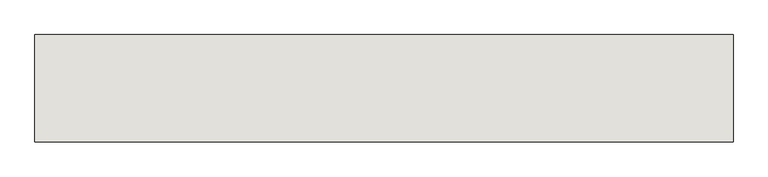
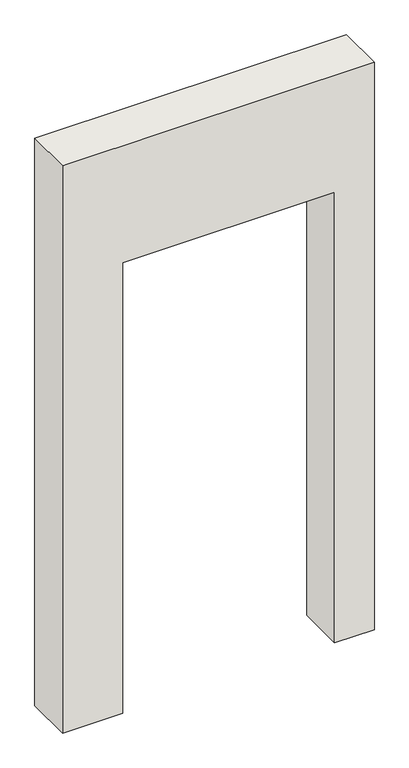
"""IFC4 building model written with IfcOpenShell, lengths in millimetres: wall geometry, Holzwand."""

from ifc_helpers import new_model, si_unit, frame, origin, place, context, project, spatial, polyline, outline, extrude, source, transform, mapped, element, save


def wall_15884945(model_context):
    return source(origin(), model_context, "Body", "SweptSolid", [
        extrude(outline(polyline([(1985.0, 1134.6134938), (0.0, 1134.6134938), (0.0, 1300.0), (2500.0, 1300.0), (2500.0, 0.0), (0.0, 0.0), (0.0, 249.6134938), (1985.0, 249.6134938), (1985.0, 1134.6134938)])), frame((0.0, 0.0, 0.0), z_axis=(0.0, 1.0, 0.0), x_axis=(0.0, 0.0, 1.0)), (0.0, 0.0, 1.0), 200.0),
    ])


if __name__ == "__main__":
    model = new_model("IFC4")
    model_context = context("Model", 3, world=origin())
    ifc_project = project(units=[si_unit("LENGTHUNIT", "METRE", prefix="MILLI")], contexts=[model_context])
    site = spatial("IfcSite", under=ifc_project)
    building = spatial("IfcBuilding", under=site)
    placement = place(None, origin())
    wall_shape = wall_15884945(model_context)
    element("IfcWall", 1, ObjectType="Holzwand", at=placement, inside=building, context=model_context, shape_type="MappedRepresentation", body=[
        mapped(wall_shape, transform((0.0, 0.0, 0.0), x_axis=(1.0, 0.0, 0.0), y_axis=(0.0, 1.0, 0.0), z_axis=(0.0, 0.0, 1.0))),
    ])
    save(model, "model.ifc")

# Revit data of these elements
# Element 1 (IfcWall, "Holzwand")
#   Materials on its faces: "holzschalung"
# Materials
#   "holzschalung": class "Unassigned", colour RGB 128 128 128, transparency 0
